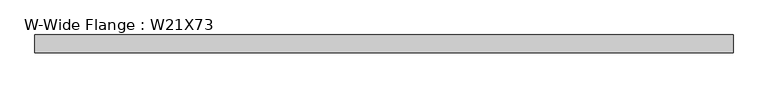
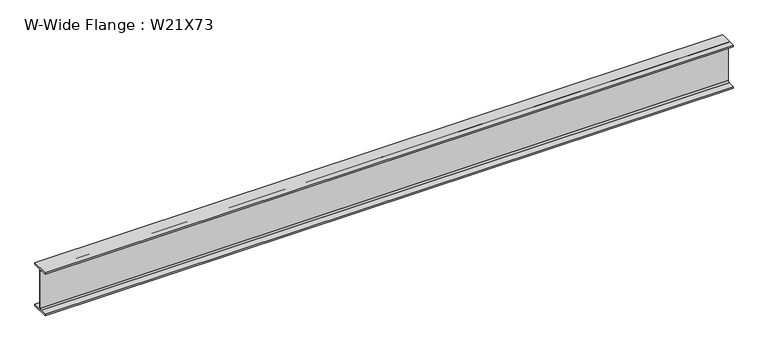
"""IFC4 building model written with IfcOpenShell, lengths in millimetres: beam geometry, W-Wide Flange : W21X73."""

from ifc_helpers import new_model, si_unit, point, frame, frame_2d, origin, place, context, project, spatial, polyline, circle_curve, trimmed, segment, composite_curve, outline, extrude, source, transform, mapped, element, save


def w_wide_flange_w21x73_f7e241f9(model_context):
    return source(origin(), model_context, "Body", "SweptSolid", [
        extrude(outline(composite_curve([segment(polyline([(105.41, -250.444), (105.41, -269.24), (-105.41, -269.24), (-105.41, -250.444), (-23.495, -250.444)]), True, "CONTINUOUS"), segment(trimmed(circle_curve(frame_2d((-23.495, -232.7275)), 17.7165), [point((-23.495, -250.444))], [point((-5.7785, -232.7275))], True, "CARTESIAN"), True, "CONTINUOUS"), segment(polyline([(-5.7785, -232.7275), (-5.7785, 232.7275)]), True, "CONTINUOUS"), segment(trimmed(circle_curve(frame_2d((-23.495, 232.7275)), 17.7165), [point((-5.7785, 232.7275))], [point((-23.495, 250.444))], True, "CARTESIAN"), True, "CONTINUOUS"), segment(polyline([(-23.495, 250.444), (-105.41, 250.444), (-105.41, 269.24), (105.41, 269.24), (105.41, 250.444), (23.495, 250.444)]), True, "CONTINUOUS"), segment(trimmed(circle_curve(frame_2d((23.495, 232.7275)), 17.7165), [point((23.495, 250.444))], [point((5.7785, 232.7275))], True, "CARTESIAN"), True, "CONTINUOUS"), segment(polyline([(5.7785, 232.7275), (5.7785, -232.7275)]), True, "CONTINUOUS"), segment(trimmed(circle_curve(frame_2d((23.495, -232.7275)), 17.7165), [point((5.7785, -232.7275))], [point((23.495, -250.444))], True, "CARTESIAN"), True, "CONTINUOUS"), segment(polyline([(23.495, -250.444), (105.41, -250.444)]), True, "CONTINUOUS")], self_intersect=False)), frame((-4076.7, 0.0, 0.0), z_axis=(1.0, 0.0, 0.0), x_axis=(0.0, 1.0, 0.0)), (0.0, 0.0, 1.0), 8153.4),
    ])


if __name__ == "__main__":
    model = new_model("IFC4")
    model_context = context("Model", 3, world=origin())
    ifc_project = project(units=[si_unit("LENGTHUNIT", "METRE", prefix="MILLI")], contexts=[model_context])
    site = spatial("IfcSite", under=ifc_project)
    building = spatial("IfcBuilding", under=site)
    placement = place(None, origin())
    w_wide_flange_w21x73_shape = w_wide_flange_w21x73_f7e241f9(model_context)
    element("IfcBeam", 1, ObjectType="W-Wide Flange : W21X73", at=placement, inside=building, context=model_context, shape_type="MappedRepresentation", body=[
        mapped(w_wide_flange_w21x73_shape, transform((0.0, 0.0, 0.0), x_axis=(1.0, 0.0, 0.0), y_axis=(0.0, 1.0, 0.0), z_axis=(0.0, 0.0, 1.0))),
    ])
    save(model, "model.ifc")

# Revit data of these elements
# Type "W-Wide Flange : W21X73"
#   Assembly Code = "B10"
#   W = 73
#   Length [instance default] = 5' - 0"
#   bf = 0' - 8.3"
#   d = 1' - 9.2"
#   k = 0' - 1 7/16"
#   k2 = 0' - 0.6975"
#   tf = 0' - 0.74"
#   tw = 0' - 0.455"
#   A = 0.149306 SF
#   Structural Material [instance default] = Steel ASTM A992
# Element 1 (IfcBeam, "W-Wide Flange : W21X73")
#   Materials on its faces: "Steel ASTM A992"
# Materials
#   "Steel ASTM A992": class "Metal", colour RGB 199 199 199, transparency 0, Description = "Structural steel 50ksi", Cost = 0
